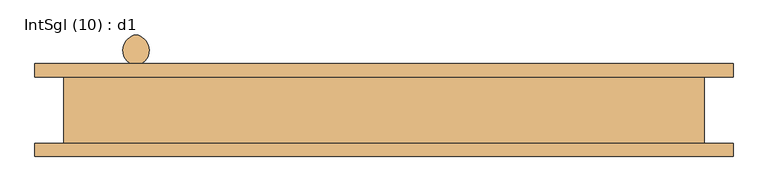
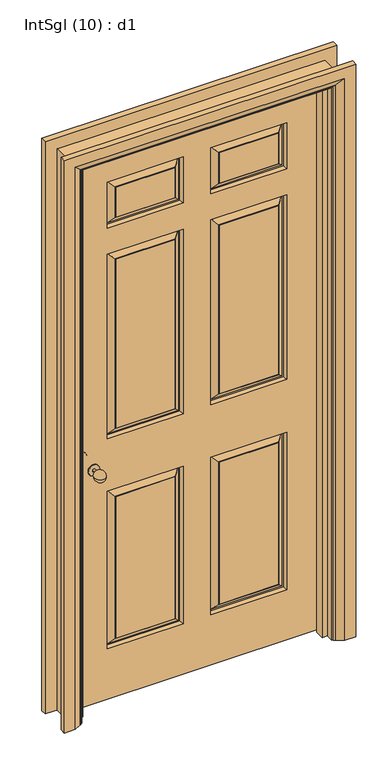
"""IFC4 building model written with IfcOpenShell, lengths in millimetres: door geometry, IntSgl (10) : d1."""

import ifcopenshell
import ifcopenshell.guid

model = None  # the IFC model being written
_history = None  # IfcOwnerHistory: only IFC2X3 demands one
_inside = {}  # id of a spatial element -> (the spatial element, [elements in it])
_under = {}  # id of a project, library or spatial element -> (it, [spatial elements below it])
_declared = {}  # id of a project -> (the project, [libraries it declares])
_typed = {}  # id of a type object -> (the type object, [elements of that type])
_made_of = {}  # id of a material, layer set ... -> (it, [elements and type objects made of it])


def new_model(schema):
    """Start an empty IFC model of exactly this schema.

    Asked for "IFC4X3", IfcOpenShell would pick the latest addendum, in which some entities
    have other attributes; the version numbers below select the first issue.
    IFC2X3 requires an IfcOwnerHistory on every rooted entity: one is made here for all.
    """
    global model, _history
    if schema == "IFC4X3":
        model = ifcopenshell.file(schema_version=(4, 3, 0, 0))
    else:
        model = ifcopenshell.file(schema=schema)
    _inside.clear()
    _under.clear()
    _declared.clear()
    _typed.clear()
    _made_of.clear()
    _history = None
    if model.schema == "IFC2X3":
        org = make("IfcOrganization", Name="unknown")
        user = make(
            "IfcPersonAndOrganization",
            ThePerson=make("IfcPerson", FamilyName="unknown"),
            TheOrganization=org,
        )
        app = make(
            "IfcApplication",
            ApplicationDeveloper=org,
            Version="unknown",
            ApplicationFullName="unknown",
            ApplicationIdentifier="unknown",
        )
        _history = make(
            "IfcOwnerHistory",
            OwningUser=user,
            OwningApplication=app,
            ChangeAction="ADDED",
            CreationDate=0,
        )
    return model


def make(cls, **values):
    """One entity of the class cls with the attributes given. An attribute that is None is left unset."""
    return model.create_entity(
        cls, **{name: value for name, value in values.items() if value is not None}
    )


def rooted(cls, **values):
    """An entity with a GlobalId (a new one), such as an element, a storey or a relation."""
    return make(cls, GlobalId=ifcopenshell.guid.new(), OwnerHistory=_history, **values)


def si_unit(unit_type, name, prefix=None):
    """IfcSIUnit, for example si_unit("LENGTHUNIT", "METRE", prefix="MILLI")."""
    return make("IfcSIUnit", UnitType=unit_type, Prefix=prefix, Name=name)


def assignment(units):
    """IfcUnitAssignment: the units of a project."""
    return None if units is None else make("IfcUnitAssignment", Units=units)


def point(xyz):
    """IfcCartesianPoint."""
    return None if xyz is None else make("IfcCartesianPoint", Coordinates=xyz)


def direction(xyz):
    """IfcDirection."""
    return None if xyz is None else make("IfcDirection", DirectionRatios=xyz)


def frame(location, z_axis=None, x_axis=None):
    """IfcAxis2Placement3D, a coordinate frame: its origin and axes. An axis left out is left unset."""
    return make(
        "IfcAxis2Placement3D",
        Location=point(location),
        Axis=direction(z_axis),
        RefDirection=direction(x_axis),
    )


def origin():
    """The frame at (0, 0, 0) with its axes left unset."""
    return frame((0.0, 0.0, 0.0))


def place(relative_to, where):
    """IfcLocalPlacement: puts the frame where relative to a parent placement (None: the world)."""
    return make(
        "IfcLocalPlacement", PlacementRelTo=relative_to, RelativePlacement=where
    )


def context(
    kind, dimensions, precision=None, world=None, true_north=None, identifier=None
):
    """IfcGeometricRepresentationContext, for example the 3D "Model" context."""
    return make(
        "IfcGeometricRepresentationContext",
        ContextIdentifier=identifier,
        ContextType=kind,
        CoordinateSpaceDimension=dimensions,
        Precision=precision,
        WorldCoordinateSystem=world,
        TrueNorth=true_north,
    )


def project(units=None, contexts=None):
    """IfcProject with its units and contexts."""
    return rooted(
        "IfcProject",
        Name="project",
        RepresentationContexts=contexts,
        UnitsInContext=assignment(units),
    )


def spatial(cls, under=None, at=None, **own):
    """A site, building, storey or space (cls), placed at a placement, below another one or the project."""
    s = rooted(cls, ObjectPlacement=at, **own)
    if under is not None:
        _under.setdefault(under.id(), (under, []))[1].append(s)
    return s


def polyline(points):
    """IfcPolyline through the points."""
    return make("IfcPolyline", Points=[point(p) for p in points])


def circle_curve(where, radius):
    """IfcCircle in the frame where."""
    return make("IfcCircle", Position=where, Radius=radius)


def ellipse_curve(where, semi_axis1, semi_axis2):
    """IfcEllipse in the frame where."""
    return make(
        "IfcEllipse", Position=where, SemiAxis1=semi_axis1, SemiAxis2=semi_axis2
    )


def trimmed(basis, trim1, trim2, sense, master):
    """IfcTrimmedCurve: the piece of a basis curve between two trims."""
    return make(
        "IfcTrimmedCurve",
        BasisCurve=basis,
        Trim1=trim1,
        Trim2=trim2,
        SenseAgreement=sense,
        MasterRepresentation=master,
    )


def outline(outer, holes=None, kind="AREA"):
    """IfcArbitraryClosedProfileDef: a profile drawn as a closed curve; with holes, ...WithVoids."""
    if holes is None:
        return make("IfcArbitraryClosedProfileDef", ProfileType=kind, OuterCurve=outer)
    return make(
        "IfcArbitraryProfileDefWithVoids",
        ProfileType=kind,
        OuterCurve=outer,
        InnerCurves=holes,
    )


def extrude(swept, where, along, depth):
    """IfcExtrudedAreaSolid: the profile swept, set in the frame where, extruded along a direction by depth."""
    return make(
        "IfcExtrudedAreaSolid",
        SweptArea=swept,
        Position=where,
        ExtrudedDirection=direction(along),
        Depth=depth,
    )


def faces_of(points, faces, orient=None, outer=None):
    """IfcFace entities. A face is a list of loops; a loop is a list of indices into points, from 0.

    orient and outer hold one flag for each loop. By default every Orientation is true, the
    first loop of a face is its IfcFaceOuterBound and the others are IfcFaceBound.
    """
    made = []
    for i, loops in enumerate(faces):
        bounds = []
        for j, loop in enumerate(loops):
            is_outer = j == 0 if outer is None else outer[i][j]
            bounds.append(
                make(
                    "IfcFaceOuterBound" if is_outer else "IfcFaceBound",
                    Bound=make("IfcPolyLoop", Polygon=[points[k] for k in loop]),
                    Orientation=True if orient is None else orient[i][j],
                )
            )
        made.append(make("IfcFace", Bounds=bounds))
    return made


def faceted_brep(points, faces, orient=None, outer=None, voids=None):
    """IfcFacetedBrep: a solid bounded by flat faces; with voids (closed shells), ...WithVoids."""
    shared = [point(p) for p in points]
    hull = make("IfcClosedShell", CfsFaces=faces_of(shared, faces, orient, outer))
    if voids is None:
        return make("IfcFacetedBrep", Outer=hull)
    return make(
        "IfcFacetedBrepWithVoids",
        Outer=hull,
        Voids=[
            make(cls, CfsFaces=faces_of(shared, fs, o, b)) for cls, fs, o, b in voids
        ],
    )


def shape(context_of_items, identifier, shape_type, items):
    """IfcShapeRepresentation: the items that make up one representation, for example the "Body"."""
    return make(
        "IfcShapeRepresentation",
        ContextOfItems=context_of_items,
        RepresentationIdentifier=identifier,
        RepresentationType=shape_type,
        Items=items,
    )


def source(mapping_origin, context_of_items, identifier, shape_type, items):
    """IfcRepresentationMap: a shape defined once, which mapped items show again and again."""
    return make(
        "IfcRepresentationMap",
        MappingOrigin=mapping_origin,
        MappedRepresentation=shape(context_of_items, identifier, shape_type, items),
    )


def transform(
    local_origin,
    x_axis=None,
    y_axis=None,
    z_axis=None,
    scale=None,
    scale2=None,
    scale3=None,
    uniform=True,
):
    """IfcCartesianTransformationOperator3D, or its non-uniform kind. x_axis, y_axis, z_axis: its Axis1, 2, 3."""
    if uniform:
        return make(
            "IfcCartesianTransformationOperator3D",
            Axis1=direction(x_axis),
            Axis2=direction(y_axis),
            LocalOrigin=point(local_origin),
            Scale=scale,
            Axis3=direction(z_axis),
        )
    return make(
        "IfcCartesianTransformationOperator3DnonUniform",
        Axis1=direction(x_axis),
        Axis2=direction(y_axis),
        LocalOrigin=point(local_origin),
        Scale=scale,
        Axis3=direction(z_axis),
        Scale2=scale2,
        Scale3=scale3,
    )


def mapped(mapping_source, mapping_target):
    """IfcMappedItem: shows the shape of a source again, moved by a transform."""
    return make(
        "IfcMappedItem", MappingSource=mapping_source, MappingTarget=mapping_target
    )


def made_of(thing, what):
    """Note that an element or type object is made of a material, layer set ...; save() writes the relation."""
    if what is not None:
        _made_of.setdefault(what.id(), (what, []))[1].append(thing)
    return thing


def element(
    cls,
    number,
    at=None,
    inside=None,
    cuts=None,
    type_object=None,
    material=None,
    context=None,
    identifier="Body",
    shape_type=None,
    held_by="IfcProductDefinitionShape",
    body=None,
    shapes=None,
    **own,
):
    """One element of the class cls, such as IfcWall. Its Tag is "e" and its number.

    at: its placement. inside: the storey or other place that contains it. cuts: it is an
    opening in that element (IfcRelVoidsElement). A single representation is given by context,
    identifier, shape_type and body (its items); several are given by shapes. held_by: the class
    of the entity that holds the representations. save() writes the other relations.
    """
    e = rooted(cls, Tag="e%d" % number, ObjectPlacement=at, **own)
    if body is not None:
        shapes = [shape(context, identifier, shape_type, body)]
    if shapes is not None:
        e.Representation = make(held_by, Representations=shapes)
    if inside is not None:
        _inside.setdefault(inside.id(), (inside, []))[1].append(e)
    if cuts is not None:
        rooted(
            "IfcRelVoidsElement", RelatingBuildingElement=cuts, RelatedOpeningElement=e
        )
    if type_object is not None:
        _typed.setdefault(type_object.id(), (type_object, []))[1].append(e)
    return made_of(e, material)


def aggregate(whole, parts):
    """IfcRelAggregates: a whole, such as a stair, and the parts it consists of."""
    return rooted("IfcRelAggregates", RelatingObject=whole, RelatedObjects=parts)


def save(model, path):
    """Write the relations noted so far, then the file.

    IfcRelAggregates (storeys below a building ...), IfcRelContainedInSpatialStructure (elements
    in a storey), IfcRelDefinesByType, IfcRelAssociatesMaterial and IfcRelDeclares: one each for
    every whole, place, type object, material and project.
    """
    for whole, parts in _under.values():
        aggregate(whole, parts)
    for where, things in _inside.values():
        rooted(
            "IfcRelContainedInSpatialStructure",
            RelatedElements=things,
            RelatingStructure=where,
        )
    for kind, things in _typed.values():
        rooted("IfcRelDefinesByType", RelatedObjects=things, RelatingType=kind)
    for what, things in _made_of.values():
        rooted("IfcRelAssociatesMaterial", RelatedObjects=things, RelatingMaterial=what)
    for by, libraries in _declared.values():
        rooted("IfcRelDeclares", RelatingContext=by, RelatedDefinitions=libraries)
    model.write(path)


def plane_surface(at):
    """IfcPlane: the flat surface through the origin of the frame at, square to its z axis."""
    return make("IfcPlane", Position=at)


def cylinder_surface(at, radius):
    """IfcCylindricalSurface: all points at the distance radius from the z axis of the frame at."""
    return make("IfcCylindricalSurface", Position=at, Radius=radius)


def revolved_surface(curve, axis_point, axis_direction):
    """IfcSurfaceOfRevolution: the curve turned about the line through axis_point along axis_direction."""
    return make(
        "IfcSurfaceOfRevolution",
        SweptCurve=make("IfcArbitraryOpenProfileDef", ProfileType="CURVE", Curve=curve),
        AxisPosition=make("IfcAxis1Placement", Location=point(axis_point), Axis=direction(axis_direction)),
    )


def advanced_brep(points, edges, surfaces, faces):
    """IfcAdvancedBrep: a solid bounded by faces that lie on surfaces and meet in shared edges.

    An edge is (start, end): straight between two places in points (the first is 0);
    or (start, end, curve); or (start, end, curve, False) where it runs against its curve.
    A face is (place in surfaces, loops), or (place, loops, False) where it looks against
    its surface's normal. A loop lists edges by number (the first is 1), with a minus sign
    where the edge is run from its end to its start. The first loop is the outer one.
    """
    corners = [point(p) for p in points]
    vertices = [make("IfcVertexPoint", VertexGeometry=c) for c in corners]
    made = []
    for start, end, *more in edges:
        made.append(
            make(
                "IfcEdgeCurve",
                EdgeStart=vertices[start],
                EdgeEnd=vertices[end],
                EdgeGeometry=more[0] if more else make("IfcPolyline", Points=[corners[start], corners[end]]),
                SameSense=more[1] if len(more) > 1 else True,
            )
        )
    hull = []
    for where, loops, *sense in faces:
        bounds = []
        for j, loop in enumerate(loops):
            ring = [make("IfcOrientedEdge", EdgeElement=made[abs(k) - 1], Orientation=k > 0) for k in loop]
            bounds.append(
                make(
                    "IfcFaceOuterBound" if j == 0 else "IfcFaceBound",
                    Bound=make("IfcEdgeLoop", EdgeList=ring),
                    Orientation=True,
                )
            )
        hull.append(make("IfcAdvancedFace", Bounds=bounds, FaceSurface=surfaces[where], SameSense=sense[0] if sense else True))
    return make("IfcAdvancedBrep", Outer=make("IfcClosedShell", CfsFaces=hull))


def intsgl_10_d1_11e9c3c5(model_context):
    return source(origin(), model_context, "Body", "SolidModel", [
        advanced_brep(
        [(-368.0, -7.0, 900.0), (-373.0, -51.437411, 900.0), (-378.0, -7.0, 900.0), (-378.0, 8.0, 900.0), (-368.0, 8.0, 900.0), (-393.0, 12.0, 900.0), (-353.0, 12.0, 900.0), (-393.0, 8.0, 900.0), (-353.0, 8.0, 900.0)],
        [
            (0, 1, circle_curve(frame((-376.1884862, -28.5786495, 900.0), z_axis=(0.0, 0.0, -1.0), x_axis=(0.0, 1.0, 0.0)), 23.0800654)),
            (1, 2, circle_curve(frame((-369.8115138, -28.5786495, 900.0), z_axis=(0.0, 0.0, -1.0), x_axis=(0.0, 1.0, 0.0)), 23.0800654)),
            (2, 0, circle_curve(frame((-373.0, -7.0, 900.0), z_axis=(0.0, -1.0, 0.0), x_axis=(-1.0, 0.0, 0.0)), 5.0)),
            (0, 2, circle_curve(frame((-373.0, -7.0, 900.0), z_axis=(0.0, -1.0, 0.0), x_axis=(-1.0, 0.0, 0.0)), 5.0)),
            (2, 3),
            (3, 4, circle_curve(frame((-373.0, 8.0, 900.0), z_axis=(0.0, -1.0, 0.0), x_axis=(-1.0, 0.0, 0.0)), 5.0)),
            (4, 0),
            (4, 3, circle_curve(frame((-373.0, 8.0, 900.0), z_axis=(0.0, -1.0, 0.0), x_axis=(-1.0, 0.0, 0.0)), 5.0)),
            (5, 6, circle_curve(frame((-373.0, 12.0, 900.0), z_axis=(0.0, 1.0, 0.0), x_axis=(1.0, 0.0, 0.0)), 20.0)),
            (6, 5, circle_curve(frame((-373.0, 12.0, 900.0), z_axis=(0.0, 1.0, 0.0), x_axis=(1.0, 0.0, 0.0)), 20.0)),
            (7, 8, circle_curve(frame((-373.0, 8.0, 900.0), z_axis=(0.0, -1.0, 0.0), x_axis=(1.0, 0.0, 0.0)), 20.0)),
            (8, 7, circle_curve(frame((-373.0, 8.0, 900.0), z_axis=(0.0, -1.0, 0.0), x_axis=(1.0, 0.0, 0.0)), 20.0)),
            (6, 8),
            (7, 5),
        ],
        [
            revolved_surface(trimmed(ellipse_curve(frame((-369.8115138, -28.5786495, 900.0), z_axis=(0.0, 0.0, -1.0), x_axis=(0.0, 1.0, 0.0)), 23.0800654, 23.0800654), [point((-373.0, -51.437411, 900.0))], [point((-378.0, -7.0, 900.0))], True, "CARTESIAN"), (-373.0, 8.0, 900.0), (0.0, 1.0, 0.0)),
            cylinder_surface(frame((-373.0, 8.0, 900.0), z_axis=(0.0, 1.0, 0.0), x_axis=(-1.0, 0.0, 0.0)), 5.0),
            plane_surface(frame((-353.0, 12.0, 900.0), z_axis=(0.0, 1.0, 0.0), x_axis=(0.0, 0.0, 1.0))),
            plane_surface(frame((-353.0, 8.0, 900.0), z_axis=(0.0, -1.0, 0.0), x_axis=(0.0, 0.0, -1.0))),
            cylinder_surface(frame((-373.0, 8.0, 900.0), z_axis=(0.0, 1.0, 0.0), x_axis=(1.0, 0.0, 0.0)), 20.0),
        ],
        [
            (0, [[1, 2, 3]]),
            (0, [[-1, 4, -2]]),
            (1, [[5, 6, 7, -3]]),
            (1, [[-7, 8, -5, -4]]),
            (2, [[9, 10]]),
            (3, [[11, 12], [-8, -6]]),
            (4, [[13, -11, 14, -10]]),
            (4, [[-14, -12, -13, -9]]),
        ],
    ),
        advanced_brep(
        [(-368.0, 69.0, 900.0), (-378.0, 69.0, 900.0), (-373.0, 113.437411, 900.0), (-368.0, 54.0, 900.0), (-378.0, 54.0, 900.0), (-393.0, 50.0, 900.0), (-353.0, 50.0, 900.0), (-393.0, 54.0, 900.0), (-353.0, 54.0, 900.0)],
        [
            (0, 1, circle_curve(frame((-373.0, 69.0, 900.0), z_axis=(0.0, 1.0, 0.0), x_axis=(-1.0, 0.0, 0.0)), 5.0)),
            (1, 2, circle_curve(frame((-369.8115138, 90.5786495, 900.0), z_axis=(0.0, 0.0, -1.0), x_axis=(0.0, -1.0, 0.0)), 23.0800654)),
            (2, 0, circle_curve(frame((-376.1884862, 90.5786495, 900.0), z_axis=(0.0, 0.0, -1.0), x_axis=(0.0, -1.0, 0.0)), 23.0800654)),
            (1, 0, circle_curve(frame((-373.0, 69.0, 900.0), z_axis=(0.0, 1.0, 0.0), x_axis=(-1.0, 0.0, 0.0)), 5.0)),
            (0, 3),
            (3, 4, circle_curve(frame((-373.0, 54.0, 900.0), z_axis=(0.0, 1.0, 0.0), x_axis=(-1.0, 0.0, 0.0)), 5.0)),
            (4, 1),
            (4, 3, circle_curve(frame((-373.0, 54.0, 900.0), z_axis=(0.0, 1.0, 0.0), x_axis=(-1.0, 0.0, 0.0)), 5.0)),
            (5, 6, circle_curve(frame((-373.0, 50.0, 900.0), z_axis=(0.0, -1.0, 0.0), x_axis=(1.0, 0.0, 0.0)), 20.0)),
            (6, 5, circle_curve(frame((-373.0, 50.0, 900.0), z_axis=(0.0, -1.0, 0.0), x_axis=(1.0, 0.0, 0.0)), 20.0)),
            (7, 8, circle_curve(frame((-373.0, 54.0, 900.0), z_axis=(0.0, 1.0, 0.0), x_axis=(1.0, 0.0, 0.0)), 20.0)),
            (8, 7, circle_curve(frame((-373.0, 54.0, 900.0), z_axis=(0.0, 1.0, 0.0), x_axis=(1.0, 0.0, 0.0)), 20.0)),
            (5, 7),
            (8, 6),
        ],
        [
            revolved_surface(trimmed(ellipse_curve(frame((-369.8115138, 90.5786495, 900.0), z_axis=(0.0, 0.0, 1.0), x_axis=(0.0, -1.0, 0.0)), 23.0800654, 23.0800654), [point((-373.0, 113.437411, 900.0))], [point((-378.0, 69.0, 900.0))], True, "CARTESIAN"), (-373.0, 54.0, 900.0), (0.0, -1.0, 0.0)),
            cylinder_surface(frame((-373.0, 54.0, 900.0), z_axis=(0.0, -1.0, 0.0), x_axis=(-1.0, 0.0, 0.0)), 5.0),
            plane_surface(frame((-353.0, 50.0, 900.0), z_axis=(0.0, -1.0, 0.0), x_axis=(0.0, 0.0, 1.0))),
            plane_surface(frame((-353.0, 54.0, 900.0), z_axis=(0.0, 1.0, 0.0), x_axis=(0.0, 0.0, -1.0))),
            cylinder_surface(frame((-373.0, 54.0, 900.0), z_axis=(0.0, -1.0, 0.0), x_axis=(1.0, 0.0, 0.0)), 20.0),
        ],
        [
            (0, [[1, 2, 3]]),
            (0, [[-2, 4, -3]]),
            (1, [[-1, 5, 6, 7]]),
            (1, [[-4, -7, 8, -5]]),
            (2, [[9, 10]]),
            (3, [[11, 12], [-6, -8]]),
            (4, [[-9, 13, -12, 14]]),
            (4, [[-10, -14, -11, -13]]),
        ],
    ),
        faceted_brep([(-448.0, 12.0, 2103.0), (-448.0, 12.0, 8.0), (448.0, 12.0, 8.0), (448.0, 12.0, 2103.0), (-50.0, 12.0, 800.0), (-50.0, 12.0, 200.0), (-323.0, 12.0, 200.0), (-323.0, 12.0, 800.0), (323.0, 12.0, 800.0), (323.0, 12.0, 200.0), (50.0, 12.0, 200.0), (50.0, 12.0, 800.0), (-50.0, 12.0, 1703.0), (-50.0, 12.0, 1000.0), (-323.0, 12.0, 1000.0), (-323.0, 12.0, 1703.0), (323.0, 12.0, 1703.0), (323.0, 12.0, 1000.0), (50.0, 12.0, 1000.0), (50.0, 12.0, 1703.0), (-50.0, 12.0, 1978.0), (-50.0, 12.0, 1803.0), (-323.0, 12.0, 1803.0), (-323.0, 12.0, 1978.0), (323.0, 12.0, 1978.0), (323.0, 12.0, 1803.0), (50.0, 12.0, 1803.0), (50.0, 12.0, 1978.0), (-80.0, 12.0, 230.0), (-80.0, 12.0, 770.0), (-293.0, 12.0, 770.0), (-293.0, 12.0, 230.0), (293.0, 12.0, 230.0), (293.0, 12.0, 770.0), (80.0, 12.0, 770.0), (80.0, 12.0, 230.0), (-80.0, 12.0, 1030.0), (-80.0, 12.0, 1673.0), (-293.0, 12.0, 1673.0), (-293.0, 12.0, 1030.0), (293.0, 12.0, 1030.0), (293.0, 12.0, 1673.0), (80.0, 12.0, 1673.0), (80.0, 12.0, 1030.0), (-80.0, 12.0, 1833.0), (-80.0, 12.0, 1948.0), (-293.0, 12.0, 1948.0), (-293.0, 12.0, 1833.0), (293.0, 12.0, 1833.0), (293.0, 12.0, 1948.0), (80.0, 12.0, 1948.0), (80.0, 12.0, 1833.0), (-448.0, 50.0, 2103.0), (448.0, 50.0, 2103.0), (448.0, 50.0, 8.0), (-448.0, 50.0, 8.0), (50.0, 50.0, 800.0), (50.0, 50.0, 200.0), (323.0, 50.0, 200.0), (323.0, 50.0, 800.0), (-323.0, 50.0, 800.0), (-323.0, 50.0, 200.0), (-50.0, 50.0, 200.0), (-50.0, 50.0, 800.0), (50.0, 50.0, 1703.0), (50.0, 50.0, 1000.0), (323.0, 50.0, 1000.0), (323.0, 50.0, 1703.0), (-323.0, 50.0, 1703.0), (-323.0, 50.0, 1000.0), (-50.0, 50.0, 1000.0), (-50.0, 50.0, 1703.0), (50.0, 50.0, 1978.0), (50.0, 50.0, 1803.0), (323.0, 50.0, 1803.0), (323.0, 50.0, 1978.0), (-323.0, 50.0, 1978.0), (-323.0, 50.0, 1803.0), (-50.0, 50.0, 1803.0), (-50.0, 50.0, 1978.0), (80.0, 50.0, 230.0), (80.0, 50.0, 770.0), (293.0, 50.0, 770.0), (293.0, 50.0, 230.0), (-293.0, 50.0, 230.0), (-293.0, 50.0, 770.0), (-80.0, 50.0, 770.0), (-80.0, 50.0, 230.0), (80.0, 50.0, 1030.0), (80.0, 50.0, 1673.0), (293.0, 50.0, 1673.0), (293.0, 50.0, 1030.0), (-293.0, 50.0, 1030.0), (-293.0, 50.0, 1673.0), (-80.0, 50.0, 1673.0), (-80.0, 50.0, 1030.0), (80.0, 50.0, 1833.0), (80.0, 50.0, 1948.0), (293.0, 50.0, 1948.0), (293.0, 50.0, 1833.0), (-293.0, 50.0, 1833.0), (-293.0, 50.0, 1948.0), (-80.0, 50.0, 1948.0), (-80.0, 50.0, 1833.0), (80.0, 49.0, 230.0), (80.0, 49.0, 770.0), (58.0, 35.0, 208.0), (58.0, 35.0, 792.0), (78.0, 49.0, 772.0), (78.0, 49.0, 228.0), (53.0, 35.0, 797.0), (53.0, 35.0, 203.0), (293.0, 49.0, 770.0), (315.0, 35.0, 792.0), (295.0, 49.0, 772.0), (320.0, 35.0, 797.0), (293.0, 49.0, 230.0), (315.0, 35.0, 208.0), (295.0, 49.0, 228.0), (320.0, 35.0, 203.0), (-293.0, 49.0, 230.0), (-293.0, 49.0, 770.0), (-315.0, 35.0, 208.0), (-315.0, 35.0, 792.0), (-295.0, 49.0, 772.0), (-295.0, 49.0, 228.0), (-320.0, 35.0, 797.0), (-320.0, 35.0, 203.0), (-80.0, 49.0, 770.0), (-58.0, 35.0, 792.0), (-78.0, 49.0, 772.0), (-53.0, 35.0, 797.0), (-80.0, 49.0, 230.0), (-58.0, 35.0, 208.0), (-78.0, 49.0, 228.0), (-53.0, 35.0, 203.0), (80.0, 49.0, 1030.0), (80.0, 49.0, 1673.0), (58.0, 35.0, 1008.0), (58.0, 35.0, 1695.0), (78.0, 49.0, 1675.0), (78.0, 49.0, 1028.0), (53.0, 35.0, 1700.0), (53.0, 35.0, 1003.0), (293.0, 49.0, 1673.0), (315.0, 35.0, 1695.0), (295.0, 49.0, 1675.0), (320.0, 35.0, 1700.0), (293.0, 49.0, 1030.0), (315.0, 35.0, 1008.0), (295.0, 49.0, 1028.0), (320.0, 35.0, 1003.0), (-293.0, 49.0, 1030.0), (-293.0, 49.0, 1673.0), (-315.0, 35.0, 1008.0), (-315.0, 35.0, 1695.0), (-295.0, 49.0, 1675.0), (-295.0, 49.0, 1028.0), (-320.0, 35.0, 1700.0), (-320.0, 35.0, 1003.0), (-80.0, 49.0, 1673.0), (-58.0, 35.0, 1695.0), (-78.0, 49.0, 1675.0), (-53.0, 35.0, 1700.0), (-80.0, 49.0, 1030.0), (-58.0, 35.0, 1008.0), (-78.0, 49.0, 1028.0), (-53.0, 35.0, 1003.0), (80.0, 49.0, 1833.0), (80.0, 49.0, 1948.0), (58.0, 35.0, 1811.0), (58.0, 35.0, 1970.0), (78.0, 49.0, 1950.0), (78.0, 49.0, 1831.0), (53.0, 35.0, 1975.0), (53.0, 35.0, 1806.0), (293.0, 49.0, 1948.0), (315.0, 35.0, 1970.0), (295.0, 49.0, 1950.0), (320.0, 35.0, 1975.0), (293.0, 49.0, 1833.0), (315.0, 35.0, 1811.0), (295.0, 49.0, 1831.0), (320.0, 35.0, 1806.0), (-293.0, 49.0, 1833.0), (-293.0, 49.0, 1948.0), (-315.0, 35.0, 1811.0), (-315.0, 35.0, 1970.0), (-295.0, 49.0, 1950.0), (-295.0, 49.0, 1831.0), (-320.0, 35.0, 1975.0), (-320.0, 35.0, 1806.0), (-80.0, 49.0, 1948.0), (-58.0, 35.0, 1970.0), (-78.0, 49.0, 1950.0), (-53.0, 35.0, 1975.0), (-80.0, 49.0, 1833.0), (-58.0, 35.0, 1811.0), (-78.0, 49.0, 1831.0), (-53.0, 35.0, 1806.0), (-80.0, 13.0, 230.0), (-80.0, 13.0, 770.0), (-58.0, 27.0, 208.0), (-58.0, 27.0, 792.0), (-78.0, 13.0, 772.0), (-78.0, 13.0, 228.0), (-53.0, 27.0, 797.0), (-53.0, 27.0, 203.0), (-293.0, 13.0, 770.0), (-315.0, 27.0, 792.0), (-295.0, 13.0, 772.0), (-320.0, 27.0, 797.0), (-293.0, 13.0, 230.0), (-315.0, 27.0, 208.0), (-295.0, 13.0, 228.0), (-320.0, 27.0, 203.0), (293.0, 13.0, 230.0), (293.0, 13.0, 770.0), (315.0, 27.0, 208.0), (315.0, 27.0, 792.0), (295.0, 13.0, 772.0), (295.0, 13.0, 228.0), (320.0, 27.0, 797.0), (320.0, 27.0, 203.0), (80.0, 13.0, 770.0), (58.0, 27.0, 792.0), (78.0, 13.0, 772.0), (53.0, 27.0, 797.0), (80.0, 13.0, 230.0), (58.0, 27.0, 208.0), (78.0, 13.0, 228.0), (53.0, 27.0, 203.0), (-80.0, 13.0, 1030.0), (-80.0, 13.0, 1673.0), (-58.0, 27.0, 1008.0), (-58.0, 27.0, 1695.0), (-78.0, 13.0, 1675.0), (-78.0, 13.0, 1028.0), (-53.0, 27.0, 1700.0), (-53.0, 27.0, 1003.0), (-293.0, 13.0, 1673.0), (-315.0, 27.0, 1695.0), (-295.0, 13.0, 1675.0), (-320.0, 27.0, 1700.0), (-293.0, 13.0, 1030.0), (-315.0, 27.0, 1008.0), (-295.0, 13.0, 1028.0), (-320.0, 27.0, 1003.0), (293.0, 13.0, 1030.0), (293.0, 13.0, 1673.0), (315.0, 27.0, 1008.0), (315.0, 27.0, 1695.0), (295.0, 13.0, 1675.0), (295.0, 13.0, 1028.0), (320.0, 27.0, 1700.0), (320.0, 27.0, 1003.0), (80.0, 13.0, 1673.0), (58.0, 27.0, 1695.0), (78.0, 13.0, 1675.0), (53.0, 27.0, 1700.0), (80.0, 13.0, 1030.0), (58.0, 27.0, 1008.0), (78.0, 13.0, 1028.0), (53.0, 27.0, 1003.0), (-80.0, 13.0, 1833.0), (-80.0, 13.0, 1948.0), (-58.0, 27.0, 1811.0), (-58.0, 27.0, 1970.0), (-78.0, 13.0, 1950.0), (-78.0, 13.0, 1831.0), (-53.0, 27.0, 1975.0), (-53.0, 27.0, 1806.0), (-293.0, 13.0, 1948.0), (-315.0, 27.0, 1970.0), (-295.0, 13.0, 1950.0), (-320.0, 27.0, 1975.0), (-293.0, 13.0, 1833.0), (-315.0, 27.0, 1811.0), (-295.0, 13.0, 1831.0), (-320.0, 27.0, 1806.0), (293.0, 13.0, 1833.0), (293.0, 13.0, 1948.0), (315.0, 27.0, 1811.0), (315.0, 27.0, 1970.0), (295.0, 13.0, 1950.0), (295.0, 13.0, 1831.0), (320.0, 27.0, 1975.0), (320.0, 27.0, 1806.0), (80.0, 13.0, 1948.0), (58.0, 27.0, 1970.0), (78.0, 13.0, 1950.0), (53.0, 27.0, 1975.0), (80.0, 13.0, 1833.0), (58.0, 27.0, 1811.0), (78.0, 13.0, 1831.0), (53.0, 27.0, 1806.0)], [[[0, 1, 2, 3], [4, 5, 6, 7], [8, 9, 10, 11], [12, 13, 14, 15], [16, 17, 18, 19], [20, 21, 22, 23], [24, 25, 26, 27]], [[28, 29, 30, 31]], [[32, 33, 34, 35]], [[36, 37, 38, 39]], [[40, 41, 42, 43]], [[44, 45, 46, 47]], [[48, 49, 50, 51]], [[52, 53, 54, 55], [56, 57, 58, 59], [60, 61, 62, 63], [64, 65, 66, 67], [68, 69, 70, 71], [72, 73, 74, 75], [76, 77, 78, 79]], [[80, 81, 82, 83]], [[84, 85, 86, 87]], [[88, 89, 90, 91]], [[92, 93, 94, 95]], [[96, 97, 98, 99]], [[100, 101, 102, 103]], [[1, 0, 52, 55]], [[2, 1, 55, 54]], [[3, 2, 54, 53]], [[0, 3, 53, 52]], [[104, 105, 81, 80]], [[106, 107, 108, 109]], [[56, 110, 111, 57]], [[81, 105, 112, 82]], [[108, 107, 113, 114]], [[110, 56, 59, 115]], [[82, 112, 116, 83]], [[114, 113, 117, 118]], [[115, 59, 58, 119]], [[104, 80, 83, 116]], [[109, 108, 114, 118], [105, 104, 116, 112]], [[106, 109, 118, 117]], [[111, 110, 115, 119], [107, 106, 117, 113]], [[57, 111, 119, 58]], [[120, 121, 85, 84]], [[122, 123, 124, 125]], [[60, 126, 127, 61]], [[85, 121, 128, 86]], [[124, 123, 129, 130]], [[126, 60, 63, 131]], [[86, 128, 132, 87]], [[130, 129, 133, 134]], [[131, 63, 62, 135]], [[120, 84, 87, 132]], [[125, 124, 130, 134], [121, 120, 132, 128]], [[122, 125, 134, 133]], [[127, 126, 131, 135], [123, 122, 133, 129]], [[61, 127, 135, 62]], [[136, 137, 89, 88]], [[138, 139, 140, 141]], [[64, 142, 143, 65]], [[89, 137, 144, 90]], [[140, 139, 145, 146]], [[142, 64, 67, 147]], [[90, 144, 148, 91]], [[146, 145, 149, 150]], [[147, 67, 66, 151]], [[136, 88, 91, 148]], [[141, 140, 146, 150], [137, 136, 148, 144]], [[138, 141, 150, 149]], [[143, 142, 147, 151], [139, 138, 149, 145]], [[65, 143, 151, 66]], [[152, 153, 93, 92]], [[154, 155, 156, 157]], [[68, 158, 159, 69]], [[93, 153, 160, 94]], [[156, 155, 161, 162]], [[158, 68, 71, 163]], [[94, 160, 164, 95]], [[162, 161, 165, 166]], [[163, 71, 70, 167]], [[152, 92, 95, 164]], [[157, 156, 162, 166], [153, 152, 164, 160]], [[154, 157, 166, 165]], [[159, 158, 163, 167], [155, 154, 165, 161]], [[69, 159, 167, 70]], [[168, 169, 97, 96]], [[170, 171, 172, 173]], [[72, 174, 175, 73]], [[97, 169, 176, 98]], [[172, 171, 177, 178]], [[174, 72, 75, 179]], [[98, 176, 180, 99]], [[178, 177, 181, 182]], [[179, 75, 74, 183]], [[168, 96, 99, 180]], [[173, 172, 178, 182], [169, 168, 180, 176]], [[170, 173, 182, 181]], [[175, 174, 179, 183], [171, 170, 181, 177]], [[73, 175, 183, 74]], [[184, 185, 101, 100]], [[186, 187, 188, 189]], [[76, 190, 191, 77]], [[101, 185, 192, 102]], [[188, 187, 193, 194]], [[190, 76, 79, 195]], [[102, 192, 196, 103]], [[194, 193, 197, 198]], [[195, 79, 78, 199]], [[184, 100, 103, 196]], [[189, 188, 194, 198], [185, 184, 196, 192]], [[186, 189, 198, 197]], [[191, 190, 195, 199], [187, 186, 197, 193]], [[77, 191, 199, 78]], [[200, 201, 29, 28]], [[202, 203, 204, 205]], [[4, 206, 207, 5]], [[29, 201, 208, 30]], [[204, 203, 209, 210]], [[206, 4, 7, 211]], [[30, 208, 212, 31]], [[210, 209, 213, 214]], [[211, 7, 6, 215]], [[200, 28, 31, 212]], [[205, 204, 210, 214], [201, 200, 212, 208]], [[202, 205, 214, 213]], [[207, 206, 211, 215], [203, 202, 213, 209]], [[5, 207, 215, 6]], [[216, 217, 33, 32]], [[218, 219, 220, 221]], [[8, 222, 223, 9]], [[33, 217, 224, 34]], [[220, 219, 225, 226]], [[222, 8, 11, 227]], [[34, 224, 228, 35]], [[226, 225, 229, 230]], [[227, 11, 10, 231]], [[216, 32, 35, 228]], [[221, 220, 226, 230], [217, 216, 228, 224]], [[218, 221, 230, 229]], [[223, 222, 227, 231], [219, 218, 229, 225]], [[9, 223, 231, 10]], [[232, 233, 37, 36]], [[234, 235, 236, 237]], [[12, 238, 239, 13]], [[37, 233, 240, 38]], [[236, 235, 241, 242]], [[238, 12, 15, 243]], [[38, 240, 244, 39]], [[242, 241, 245, 246]], [[243, 15, 14, 247]], [[232, 36, 39, 244]], [[237, 236, 242, 246], [233, 232, 244, 240]], [[234, 237, 246, 245]], [[239, 238, 243, 247], [235, 234, 245, 241]], [[13, 239, 247, 14]], [[248, 249, 41, 40]], [[250, 251, 252, 253]], [[16, 254, 255, 17]], [[41, 249, 256, 42]], [[252, 251, 257, 258]], [[254, 16, 19, 259]], [[42, 256, 260, 43]], [[258, 257, 261, 262]], [[259, 19, 18, 263]], [[248, 40, 43, 260]], [[253, 252, 258, 262], [249, 248, 260, 256]], [[250, 253, 262, 261]], [[255, 254, 259, 263], [251, 250, 261, 257]], [[17, 255, 263, 18]], [[264, 265, 45, 44]], [[266, 267, 268, 269]], [[20, 270, 271, 21]], [[45, 265, 272, 46]], [[268, 267, 273, 274]], [[270, 20, 23, 275]], [[46, 272, 276, 47]], [[274, 273, 277, 278]], [[275, 23, 22, 279]], [[264, 44, 47, 276]], [[269, 268, 274, 278], [265, 264, 276, 272]], [[266, 269, 278, 277]], [[271, 270, 275, 279], [267, 266, 277, 273]], [[21, 271, 279, 22]], [[280, 281, 49, 48]], [[282, 283, 284, 285]], [[24, 286, 287, 25]], [[49, 281, 288, 50]], [[284, 283, 289, 290]], [[286, 24, 27, 291]], [[50, 288, 292, 51]], [[290, 289, 293, 294]], [[291, 27, 26, 295]], [[280, 48, 51, 292]], [[285, 284, 290, 294], [281, 280, 292, 288]], [[282, 285, 294, 293]], [[287, 286, 291, 295], [283, 282, 293, 289]], [[25, 287, 295, 26]]]),
        advanced_brep(
        [(525.0, 70.0, 0.0), (525.0, 50.0, 0.0), (455.0, 50.0, 0.0), (459.0, 56.0, 0.0), (485.0, 70.0, 0.0), (525.0, 70.0, 2180.0), (525.0, 50.0, 2180.0), (-525.0, 50.0, 2180.0), (-525.0, 50.0, 0.0), (-455.0, 50.0, 0.0), (-455.0, 50.0, 2110.0), (455.0, 50.0, 2110.0), (459.0, 56.0, 2114.0), (485.0, 70.0, 2140.0), (-485.0, 70.0, 2140.0), (-485.0, 70.0, 0.0), (-525.0, 70.0, 0.0), (-525.0, 70.0, 2180.0), (-459.0, 56.0, 0.0), (-459.0, 56.0, 2114.0)],
        [
            (0, 1),
            (1, 2),
            (2, 3, circle_curve(frame((463.0, 49.0, 0.0), z_axis=(0.0, 0.0, -1.0), x_axis=(1.0, 0.0, 0.0)), 8.0622577)),
            (3, 4),
            (4, 0),
            (0, 5),
            (5, 6),
            (6, 1),
            (6, 7),
            (7, 8),
            (8, 9),
            (9, 10),
            (10, 11),
            (11, 2),
            (11, 12, ellipse_curve(frame((463.0, 49.0, 2118.0), z_axis=(0.7071067811865475, 0.0, -0.7071067811865475), x_axis=(-0.7071067811865474, 0.0, -0.7071067811865476)), 11.4017543, 8.0622577)),
            (12, 3),
            (12, 13),
            (13, 4),
            (13, 14),
            (14, 15),
            (15, 16),
            (16, 17),
            (17, 5),
            (7, 17),
            (16, 8),
            (15, 18),
            (18, 9, circle_curve(frame((-463.0, 49.0, 0.0), z_axis=(0.0, 0.0, -1.0), x_axis=(-1.0, 0.0, 0.0)), 8.0622577)),
            (19, 10, ellipse_curve(frame((-463.0, 49.0, 2118.0), z_axis=(-0.7071067811865475, 0.0, -0.7071067811865475), x_axis=(-0.7071067811865474, 0.0, 0.7071067811865476)), 11.4017543, 8.0622577)),
            (18, 19),
            (14, 19),
            (19, 12),
        ],
        [
            plane_surface(frame((455.0, 50.0, 0.0), z_axis=(0.0, 0.0, -1.0), x_axis=(0.0, 1.0, 0.0))),
            plane_surface(frame((525.0, 70.0, 0.0), z_axis=(1.0, 0.0, 0.0), x_axis=(0.0, 0.0, 1.0))),
            plane_surface(frame((525.0, 50.0, 0.0), z_axis=(0.0, -1.0, 0.0), x_axis=(0.0, 0.0, 1.0))),
            cylinder_surface(frame((463.0, 49.0, 0.0), z_axis=(0.0, 0.0, -1.0), x_axis=(1.0, 0.0, 0.0)), 8.0622577),
            plane_surface(frame((459.0, 56.0, 0.0), z_axis=(-0.4740998230350183, 0.8804710999221749, 0.0), x_axis=(0.0, 0.0, 1.0))),
            plane_surface(frame((485.0, 70.0, 0.0), z_axis=(0.0, 1.0, 0.0), x_axis=(0.0, 0.0, 1.0))),
            plane_surface(frame((-525.0, 70.0, 2180.0), z_axis=(-1.0, 0.0, 0.0), x_axis=(0.0, 0.0, -1.0))),
            plane_surface(frame((-455.0, 50.0, 0.0), z_axis=(0.0, 0.0, -1.0), x_axis=(0.0, 1.0, 0.0))),
            cylinder_surface(frame((-463.0, 49.0, 2110.0), z_axis=(0.0, 0.0, 1.0), x_axis=(-1.0, 0.0, 0.0)), 8.0622577),
            plane_surface(frame((-459.0, 56.0, 2114.0), z_axis=(0.4740998230350183, 0.8804710999221749, 0.0), x_axis=(0.0, 0.0, -1.0))),
            plane_surface(frame((525.0, 70.0, 2180.0), z_axis=(0.0, 0.0, 1.0), x_axis=(-1.0, 0.0, 0.0))),
            cylinder_surface(frame((455.0, 49.0, 2118.0), z_axis=(1.0, 0.0, 0.0), x_axis=(0.0, 0.0, 1.0)), 8.0622577),
            plane_surface(frame((459.0, 56.0, 2114.0), z_axis=(0.0, 0.8804710999221749, -0.4740998230350183), x_axis=(-1.0, 0.0, 0.0))),
        ],
        [
            (0, [[1, 2, 3, 4, 5]]),
            (1, [[-1, 6, 7, 8]]),
            (2, [[-2, -8, 9, 10, 11, 12, 13, 14]]),
            (3, [[-3, -14, 15, 16]]),
            (4, [[-4, -16, 17, 18]]),
            (5, [[-5, -18, 19, 20, 21, 22, 23, -6]]),
            (6, [[24, -22, 25, -10]]),
            (7, [[-21, 26, 27, -11, -25]]),
            (8, [[28, -12, -27, 29]]),
            (9, [[30, -29, -26, -20]]),
            (10, [[-7, -23, -24, -9]]),
            (11, [[-15, -13, -28, 31]]),
            (12, [[-17, -31, -30, -19]]),
        ],
    ),
        advanced_brep(
        [(-525.0, -70.0, 0.0), (-525.0, -50.0, 0.0), (-455.0, -50.0, 0.0), (-459.0, -56.0, 0.0), (-485.0, -70.0, 0.0), (-525.0, -70.0, 2180.0), (-525.0, -50.0, 2180.0), (525.0, -50.0, 2180.0), (525.0, -50.0, 0.0), (455.0, -50.0, 0.0), (455.0, -50.0, 2110.0), (-455.0, -50.0, 2110.0), (-459.0, -56.0, 2114.0), (-485.0, -70.0, 2140.0), (485.0, -70.0, 2140.0), (485.0, -70.0, 0.0), (525.0, -70.0, 0.0), (525.0, -70.0, 2180.0), (459.0, -56.0, 0.0), (459.0, -56.0, 2114.0)],
        [
            (0, 1),
            (1, 2),
            (2, 3, circle_curve(frame((-463.0, -49.0, 0.0), z_axis=(0.0, 0.0, -1.0), x_axis=(-1.0, 0.0, 0.0)), 8.0622577)),
            (3, 4),
            (4, 0),
            (0, 5),
            (5, 6),
            (6, 1),
            (6, 7),
            (7, 8),
            (8, 9),
            (9, 10),
            (10, 11),
            (11, 2),
            (11, 12, ellipse_curve(frame((-463.0, -49.0, 2118.0), z_axis=(-0.7071067811865475, 0.0, -0.7071067811865475), x_axis=(0.7071067811865474, 0.0, -0.7071067811865476)), 11.4017543, 8.0622577)),
            (12, 3),
            (12, 13),
            (13, 4),
            (13, 14),
            (14, 15),
            (15, 16),
            (16, 17),
            (17, 5),
            (7, 17),
            (16, 8),
            (15, 18),
            (18, 9, circle_curve(frame((463.0, -49.0, 0.0), z_axis=(0.0, 0.0, -1.0), x_axis=(1.0, 0.0, 0.0)), 8.0622577)),
            (19, 10, ellipse_curve(frame((463.0, -49.0, 2118.0), z_axis=(0.7071067811865475, 0.0, -0.7071067811865475), x_axis=(0.7071067811865474, 0.0, 0.7071067811865476)), 11.4017543, 8.0622577)),
            (18, 19),
            (14, 19),
            (19, 12),
        ],
        [
            plane_surface(frame((-455.0, -50.0, 0.0), z_axis=(0.0, 0.0, -1.0), x_axis=(0.0, -1.0, 0.0))),
            plane_surface(frame((-525.0, -70.0, 0.0), z_axis=(-1.0, 0.0, 0.0), x_axis=(0.0, 0.0, 1.0))),
            plane_surface(frame((-525.0, -50.0, 0.0), z_axis=(0.0, 1.0, 0.0), x_axis=(0.0, 0.0, 1.0))),
            cylinder_surface(frame((-463.0, -49.0, 0.0), z_axis=(0.0, 0.0, -1.0), x_axis=(-1.0, 0.0, 0.0)), 8.0622577),
            plane_surface(frame((-459.0, -56.0, 0.0), z_axis=(0.4740998230350183, -0.8804710999221749, 0.0), x_axis=(0.0, 0.0, 1.0))),
            plane_surface(frame((-485.0, -70.0, 0.0), z_axis=(0.0, -1.0, 0.0), x_axis=(0.0, 0.0, 1.0))),
            plane_surface(frame((525.0, -70.0, 2180.0), z_axis=(1.0, 0.0, 0.0), x_axis=(0.0, 0.0, -1.0))),
            plane_surface(frame((455.0, -50.0, 0.0), z_axis=(0.0, 0.0, -1.0), x_axis=(0.0, -1.0, 0.0))),
            cylinder_surface(frame((463.0, -49.0, 2110.0), z_axis=(0.0, 0.0, 1.0), x_axis=(1.0, 0.0, 0.0)), 8.0622577),
            plane_surface(frame((459.0, -56.0, 2114.0), z_axis=(-0.4740998230350183, -0.8804710999221749, 0.0), x_axis=(0.0, 0.0, -1.0))),
            plane_surface(frame((-525.0, -70.0, 2180.0), z_axis=(0.0, 0.0, 1.0), x_axis=(1.0, 0.0, 0.0))),
            cylinder_surface(frame((-455.0, -49.0, 2118.0), z_axis=(-1.0, 0.0, 0.0), x_axis=(0.0, 0.0, 1.0)), 8.0622577),
            plane_surface(frame((-459.0, -56.0, 2114.0), z_axis=(0.0, -0.8804710999221749, -0.4740998230350183), x_axis=(1.0, 0.0, 0.0))),
        ],
        [
            (0, [[1, 2, 3, 4, 5]]),
            (1, [[-1, 6, 7, 8]]),
            (2, [[-2, -8, 9, 10, 11, 12, 13, 14]]),
            (3, [[-3, -14, 15, 16]]),
            (4, [[-4, -16, 17, 18]]),
            (5, [[-5, -18, 19, 20, 21, 22, 23, -6]]),
            (6, [[24, -22, 25, -10]]),
            (7, [[-21, 26, 27, -11, -25]]),
            (8, [[28, -12, -27, 29]]),
            (9, [[30, -29, -26, -20]]),
            (10, [[-7, -23, -24, -9]]),
            (11, [[-15, -13, -28, 31]]),
            (12, [[-17, -31, -30, -19]]),
        ],
    ),
        extrude(outline(polyline([(0.0, -450.0), (0.0, -431.0), (2086.0, -431.0), (2086.0, 431.0), (0.0, 431.0), (0.0, 450.0), (2105.0, 450.0), (2105.0, -450.0), (0.0, -450.0)])), frame((0.0, -22.0, 0.0), z_axis=(0.0, 1.0, 0.0), x_axis=(0.0, 0.0, 1.0)), (0.0, 0.0, 1.0), 32.0),
        faceted_brep([(-450.0, 50.0, 0.0), (-450.0, -50.0, 0.0), (-482.0, -50.0, 0.0), (-482.0, 50.0, 0.0), (-450.0, 50.0, 2105.0), (-450.0, -50.0, 2105.0), (-482.0, -50.0, 2137.0), (-482.0, 50.0, 2137.0), (450.0, 50.0, 0.0), (482.0, 50.0, 0.0), (482.0, -50.0, 0.0), (450.0, -50.0, 0.0), (450.0, 50.0, 2105.0), (482.0, 50.0, 2137.0), (482.0, -50.0, 2137.0), (450.0, -50.0, 2105.0)], [[[0, 1, 2, 3]], [[1, 0, 4, 5]], [[2, 1, 5, 6]], [[3, 2, 6, 7]], [[0, 3, 7, 4]], [[8, 9, 10, 11]], [[12, 13, 9, 8]], [[13, 14, 10, 9]], [[14, 15, 11, 10]], [[15, 12, 8, 11]], [[5, 4, 12, 15]], [[6, 5, 15, 14]], [[7, 6, 14, 13]], [[4, 7, 13, 12]]]),
    ])


if __name__ == "__main__":
    model = new_model("IFC4")
    model_context = context("Model", 3, world=origin())
    ifc_project = project(units=[si_unit("LENGTHUNIT", "METRE", prefix="MILLI")], contexts=[model_context])
    site = spatial("IfcSite", under=ifc_project)
    building = spatial("IfcBuilding", under=site)
    placement = place(None, origin())
    intsgl_10_d1_shape = intsgl_10_d1_11e9c3c5(model_context)
    element("IfcDoor", 1, ObjectType="IntSgl (10) : d1", at=placement, inside=building, context=model_context, shape_type="MappedRepresentation", body=[
        mapped(intsgl_10_d1_shape, transform((0.0, 0.0, 0.0), x_axis=(1.0, 0.0, 0.0), y_axis=(0.0, 1.0, 0.0), z_axis=(0.0, 0.0, 1.0))),
    ])
    save(model, "model.ifc")

# Revit data of these elements
# Type "IntSgl (10) : d1"
#   Type Mark = "11"
#   Type Comments = "Internal Single"
#   Operation = "SingleSwingRight"
#   Manufacturer = "Revit"
#   Keynote = "L20"
#   Description = "Internal Single Door"
#   UnderCut = 8 mm
#   Tolerance = 2 mm
#   Thickness = 38 mm
#   Structural Tolerance = 8 mm
#   StopDepth = 32 mm
#   Stop Thickness = 19 mm
#   Stile Top Rail = 125 mm
#   Stile Shutting = 125 mm
#   Stile Muntin Rail = 100 mm
#   Stile Lock Rail = 200 mm
#   Stile Intermediate/Frieze = 100 mm
#   Stile Hanging = 125 mm
#   Stile Bottom Rail = 200 mm
#   Rough Width = 980 mm
#   Rough Height = 2145 mm
#   Height to Top Lock Rail = 1000 mm
#   Handle Z Distance = 900 mm
#   Handle X Distance = 75 mm
#   Frame Thickness = 32 mm
#   Door Panel Width = 896 mm
#   Height = 2145 mm
#   Width = 980 mm
#   Door Panel Thickness = 38 mm
#   Door Panel Offset = 0 mm
#   Door Panel Height = 2095 mm
#   Architrave Setback = 5 mm
#   Vis - Ironmongery = yes
#   Material Ironmongery = Door - Handle
#   Material Frame = Door - Frame/Mullion
#   Material Door = Door - Panel
#   Material Architrave = Door - Architrave
#   Function = (empty or 0)
#   Wall Closure = (empty or 0)
# Element 1 (IfcDoor, "IntSgl (10) : d1")
#   Materials on its faces: "Door - Panel", "Door - Architrave", "Door - Frame/Mullion", "Door - Handle"
# Materials
#   "Door - Handle": class "Miscellaneous", colour RGB 247 247 247, transparency 0
#   "Door - Frame/Mullion": class "Wood", colour RGB 212 179 113, transparency 0
#   "Door - Panel": class "Wood", colour RGB 210 159 95, transparency 0
#   "Door - Architrave": class "Wood", colour RGB 154 90 5, transparency 0
